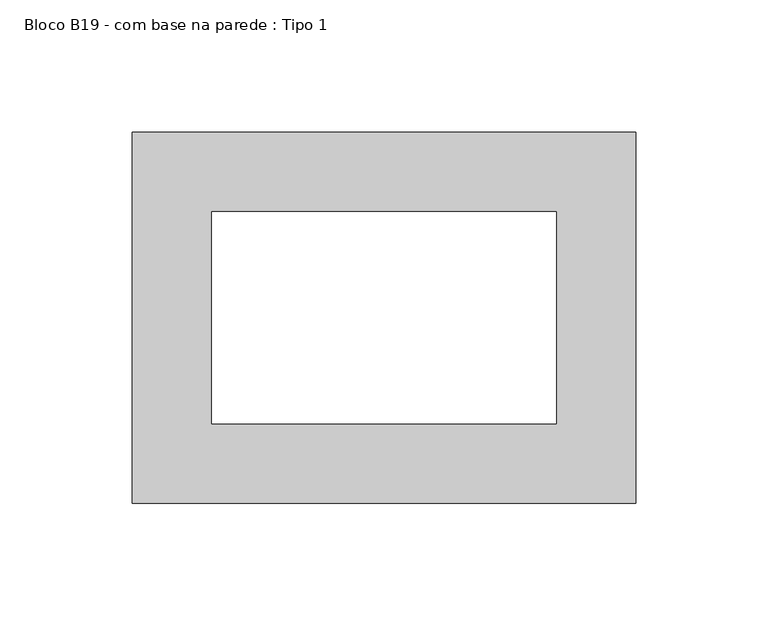
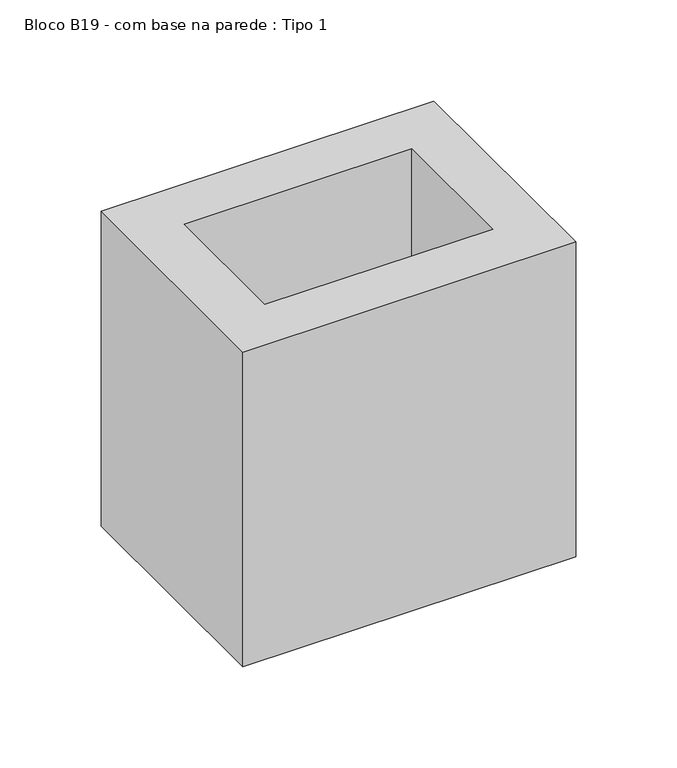
"""IFC4 building model written with IfcOpenShell, lengths in millimetres: proxy geometry, Bloco B19 - com base na parede : Tipo 1."""

from ifc_helpers import new_model, si_unit, origin, origin_with_axes, place, context, project, spatial, polyline, outline, extrude, source, transform, mapped, element, save


def bloco_b19_com_base_na_parede_tipo_1_287b7b49(model_context):
    return source(origin(), model_context, "Body", "SweptSolid", [
        extrude(outline(polyline([(220.0, -70.0), (30.0, -70.0), (30.0, 70.0), (220.0, 70.0), (220.0, -70.0)]), holes=[polyline([(60.0, -40.0), (190.0, -40.0), (190.0, 40.0), (60.0, 40.0), (60.0, -40.0)])]), origin_with_axes(), (0.0, 0.0, 1.0), 190.0),
    ])


if __name__ == "__main__":
    model = new_model("IFC4")
    model_context = context("Model", 3, world=origin())
    ifc_project = project(units=[si_unit("LENGTHUNIT", "METRE", prefix="MILLI")], contexts=[model_context])
    site = spatial("IfcSite", under=ifc_project)
    building = spatial("IfcBuilding", under=site)
    placement = place(None, origin())
    bloco_b19_com_base_na_parede_tipo_1_shape = bloco_b19_com_base_na_parede_tipo_1_287b7b49(model_context)
    element("IfcBuildingElementProxy", 1, Name="Bloco B19 - com base na parede : Tipo 1", ObjectType="Bloco B19 - com base na parede : Tipo 1", at=placement, inside=building, context=model_context, shape_type="MappedRepresentation", body=[
        mapped(bloco_b19_com_base_na_parede_tipo_1_shape, transform((0.0, 0.0, 0.0), x_axis=(1.0, 0.0, 0.0), y_axis=(0.0, 1.0, 0.0), z_axis=(0.0, 0.0, 1.0))),
    ])
    save(model, "model.ifc")

# Revit data of these elements
# Type "Bloco B19 - com base na parede : Tipo 1"
#   SINAPI = ""
#   Assembly Code = ""
